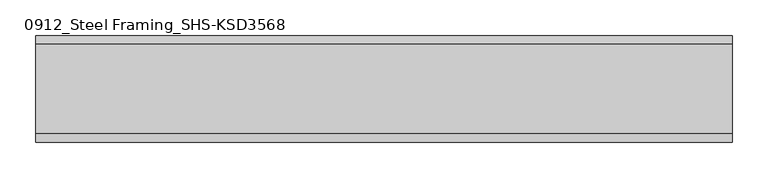
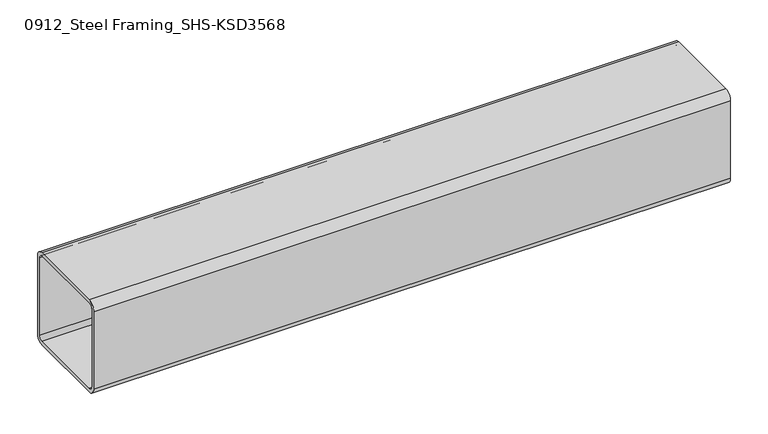
"""IFC4 building model written with IfcOpenShell, lengths in millimetres: beam geometry, 0912_Steel Framing_SHS-KSD3568 : H_SB_ASB_SHS-150x150x6."""

from ifc_helpers import new_model, si_unit, point, frame, frame_2d, origin, place, context, project, spatial, polyline, circle_curve, trimmed, segment, composite_curve, outline, extrude, source, transform, mapped, element, save


def beam_0912_steel_framing_shs_ksd3568_e9f13fd5(model_context):
    return source(origin(), model_context, "Body", "SweptSolid", [
        extrude(outline(composite_curve([segment(trimmed(circle_curve(frame_2d((-63.0, 63.0)), 12.0), [point((-75.0, 63.0))], [point((-63.0, 75.0))], False, "CARTESIAN"), True, "CONTINUOUS"), segment(polyline([(-63.0, 75.0), (63.0, 75.0)]), True, "CONTINUOUS"), segment(trimmed(circle_curve(frame_2d((63.0, 63.0)), 12.0), [point((63.0, 75.0))], [point((75.0, 63.0))], False, "CARTESIAN"), True, "CONTINUOUS"), segment(polyline([(75.0, 63.0), (75.0, -63.0)]), True, "CONTINUOUS"), segment(trimmed(circle_curve(frame_2d((63.0, -63.0)), 12.0), [point((75.0, -63.0))], [point((63.0, -75.0))], False, "CARTESIAN"), True, "CONTINUOUS"), segment(polyline([(63.0, -75.0), (-63.0, -75.0)]), True, "CONTINUOUS"), segment(trimmed(circle_curve(frame_2d((-63.0, -63.0)), 12.0), [point((-63.0, -75.0))], [point((-75.0, -63.0))], False, "CARTESIAN"), True, "CONTINUOUS"), segment(polyline([(-75.0, -63.0), (-75.0, 63.0)]), True, "CONTINUOUS")], self_intersect=False), holes=[composite_curve([segment(polyline([(63.0, 69.0), (-63.0, 69.0)]), True, "CONTINUOUS"), segment(trimmed(circle_curve(frame_2d((-63.0, 63.0)), 6.0), [point((-63.0, 69.0))], [point((-69.0, 63.0))], True, "CARTESIAN"), True, "CONTINUOUS"), segment(polyline([(-69.0, 63.0), (-69.0, -63.0)]), True, "CONTINUOUS"), segment(trimmed(circle_curve(frame_2d((-63.0, -63.0)), 6.0), [point((-69.0, -63.0))], [point((-63.0, -69.0))], True, "CARTESIAN"), True, "CONTINUOUS"), segment(polyline([(-63.0, -69.0), (63.0, -69.0)]), True, "CONTINUOUS"), segment(trimmed(circle_curve(frame_2d((63.0, -63.0)), 6.0), [point((63.0, -69.0))], [point((69.0, -63.0))], True, "CARTESIAN"), True, "CONTINUOUS"), segment(polyline([(69.0, -63.0), (69.0, 63.0)]), True, "CONTINUOUS"), segment(trimmed(circle_curve(frame_2d((63.0, 63.0)), 6.0), [point((69.0, 63.0))], [point((63.0, 69.0))], True, "CARTESIAN"), True, "CONTINUOUS")], self_intersect=False)]), frame((-490.0, 0.0, 0.0), z_axis=(1.0, 0.0, 0.0), x_axis=(0.0, 1.0, 0.0)), (0.0, 0.0, 1.0), 980.0),
    ])


if __name__ == "__main__":
    model = new_model("IFC4")
    model_context = context("Model", 3, world=origin())
    ifc_project = project(units=[si_unit("LENGTHUNIT", "METRE", prefix="MILLI")], contexts=[model_context])
    site = spatial("IfcSite", under=ifc_project)
    building = spatial("IfcBuilding", under=site)
    placement = place(None, origin())
    beam_0912_steel_framing_shs_ksd3568_shape = beam_0912_steel_framing_shs_ksd3568_e9f13fd5(model_context)
    element("IfcBeam", 1, ObjectType="0912_Steel Framing_SHS-KSD3568 : H_SB_ASB_SHS-150x150x6", at=placement, inside=building, context=model_context, shape_type="MappedRepresentation", body=[
        mapped(beam_0912_steel_framing_shs_ksd3568_shape, transform((0.0, 0.0, 0.0), x_axis=(1.0, 0.0, 0.0), y_axis=(0.0, 1.0, 0.0), z_axis=(0.0, 0.0, 1.0))),
    ])
    save(model, "model.ifc")

# Revit data of these elements
# Type "0912_Steel Framing_SHS-KSD3568 : H_SB_ASB_SHS-150x150x6"
#   H_WM Code_1 = "S01AA002-00001 | Main Steel Structure Fabrication Work | Shelter/Building | Medium Steel - Standard (90KG/M>Weight≥30KG/M) | Material: (   )"
#   H_WM Code_2 = "S03AA028-00001 | Main Steel Structure Erection Work | Shelter/Building | Medium Steel (90KG/M>Weight≥30KG/M) | Material: (   )"
#   H_WM Code_3 = "S01AA010-00001 | Main Steel Structure Fabrication Work | Shelter/Building | Steel Painting/Coating | for Non-Fireproofed Steel Surface, Surface Preparation, Primer, Second & Final Coat | Material: (   )"
#   H_Q'ty Cal Type Tag = "SB-Q2"
#   Perimeter = 0.60 m²/m
#   Nominal Weight = 26.40 kgf/m
#   Length [instance default] = 1.0000 m
#   b = 0.1500 m
#   h = 0.1500 m
#   tr = 0.0120 m
#   t = 0.0060 m
#   A = 28.36 m²
#   Structural Material [instance default] = Steel, 45-345
# Element 1 (IfcBeam, "0912_Steel Framing_SHS-KSD3568 : H_SB_ASB_SHS-150x150x6")
#   Structural Material = none
# Materials
#   "Steel, 45-345": class "Metal", colour RGB 189 187 185, transparency 0, Description = "Steel 345 MPa", Cost = 0
